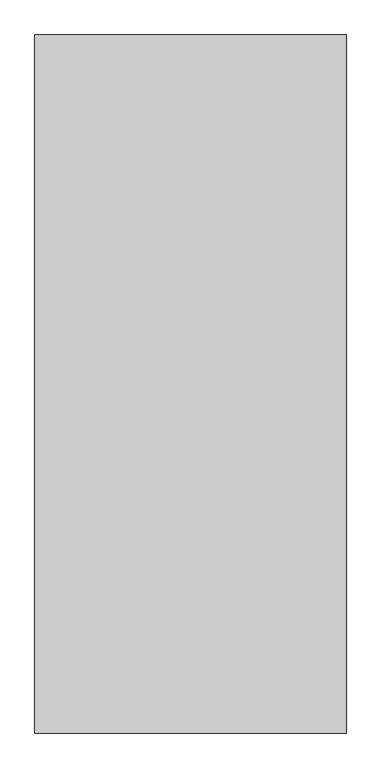
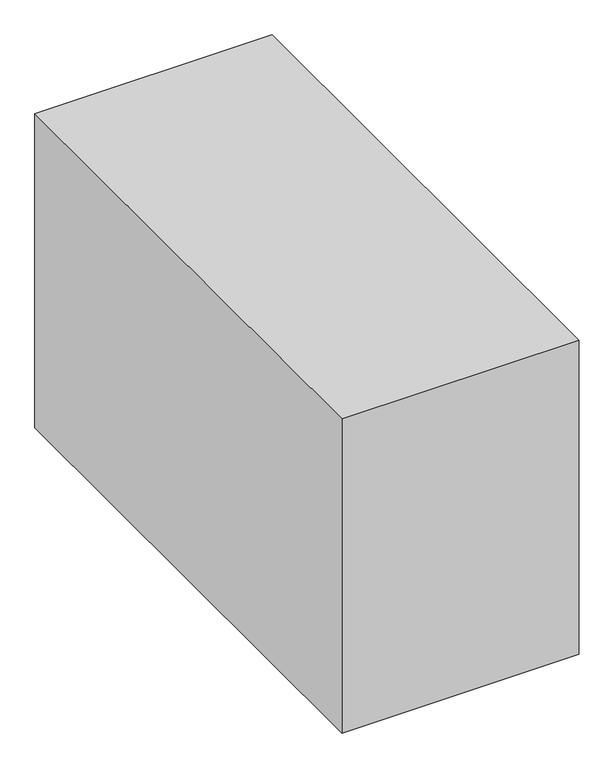
"""IFC4 building model written with IfcOpenShell, lengths in millimetres: proxy geometry, Space Planning Box_hec : Space Planning Box_hec."""

from ifc_helpers import new_model, si_unit, origin, origin_with_axes, place, context, project, spatial, polyline, outline, extrude, source, transform, mapped, element, save


def generic_models_6c75c912(model_context):
    return source(origin(), model_context, "Body", "SweptSolid", [
        extrude(outline(polyline([(1250.0, 2800.0), (1250.0, -2800.0), (-1250.0, -2800.0), (-1250.0, 2800.0), (1250.0, 2800.0)])), origin_with_axes(), (0.0, 0.0, 1.0), 3500.0),
    ])


if __name__ == "__main__":
    model = new_model("IFC4")
    model_context = context("Model", 3, world=origin())
    ifc_project = project(units=[si_unit("LENGTHUNIT", "METRE", prefix="MILLI")], contexts=[model_context])
    site = spatial("IfcSite", under=ifc_project)
    building = spatial("IfcBuilding", under=site)
    placement = place(None, origin())
    generic_models_shape = generic_models_6c75c912(model_context)
    element("IfcBuildingElementProxy", 1, Name="Space Planning Box_hec : Space Planning Box_hec", ObjectType="Space Planning Box_hec : Space Planning Box_hec", at=placement, inside=building, context=model_context, shape_type="MappedRepresentation", body=[
        mapped(generic_models_shape, transform((0.0, 0.0, 0.0), x_axis=(1.0, 0.0, 0.0), y_axis=(0.0, 1.0, 0.0), z_axis=(0.0, 0.0, 1.0))),
    ])
    save(model, "model.ifc")

# Revit data of these elements
# Type "Space Planning Box_hec : Space Planning Box_hec"
#   Type Comments = "..."
#   Room Name [instance default] = "?"
#   Interior Finish [instance default] = ""
#   Exterior Finish [instance default] = ""
#   Department [instance default] = ""
#   Assembly Code = "..."
#   ceiling height [instance default] = 0
#   Width [instance default] = 1524 mm
#   Program Area [instance default] = 0.00 m²
#   Length [instance default] = 1524 mm
#   Height [instance default] = 1524 mm
#   Area [instance default] = 2.32258 m²
#   Fill Color [instance default] = Cyan
#   Default Elevation = 0
# Element 1 (IfcBuildingElementProxy, "Space Planning Box_hec : Space Planning Box_hec")
#   Room Name = "Shower"
#   Exterior Finish = "RF1..N/A,,EW2..N/A..N/A"
#   Department = "AR"
#   Width = 2500 mm
#   Program Area = 14.00 m²
#   Length = 5600 mm
#   Height = 3500 mm
#   Area = 14.00 m²
#   Materials on its faces: "Cyan"
# Materials
#   "Cyan": class "Generic", colour RGB 0 255 255, transparency 0.2, Cost = 0
